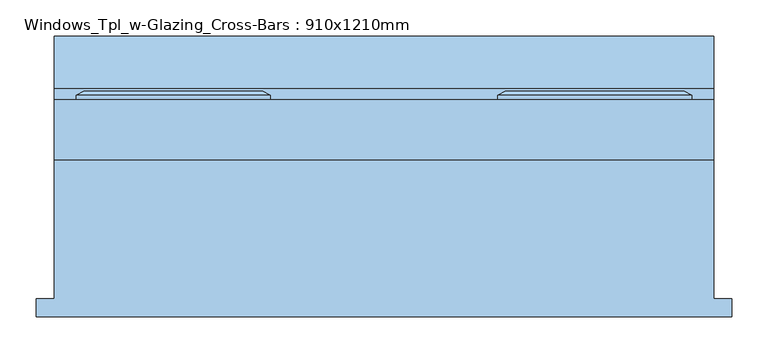
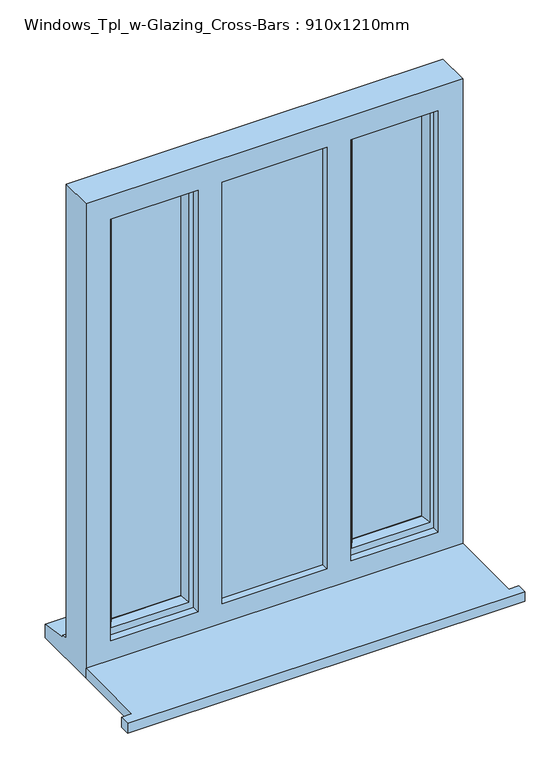
"""IFC4 building model written with IfcOpenShell, lengths in millimetres: window geometry, Windows_Tpl_w-Glazing_Cross-Bars : 910x1210mm."""

from ifc_helpers import new_model, si_unit, frame, origin, place, context, project, spatial, polyline, outline, extrude, faceted_brep, source, transform, mapped, element, save


def windows_tpl_w_glazing_cross_bars_910x1210mm_b9cba8ba(model_context):
    return source(origin(), model_context, "Body", "SolidModel", [
        extrude(outline(polyline([(-906.6666667, -178.7934322), (-906.6666667, -153.7934322), (-881.6666667, -153.7934322), (-881.6666667, 37.7065678), (28.3333333, 37.7065678), (28.3333333, -153.7934322), (53.3333333, -153.7934322), (53.3333333, -178.7934322), (-906.6666667, -178.7934322)])), frame((0.0, 0.0, 900.0), z_axis=(0.0, 0.0, 1.0), x_axis=(1.0, 0.0, 0.0)), (0.0, 0.0, 1.0), 25.0),
        extrude(outline(polyline([(-623.3333333, 72.4565678), (-811.6666667, 72.4565678), (-811.6666667, 96.4565678), (-623.3333333, 96.4565678), (-623.3333333, 72.4565678)])), frame((0.0, 0.0, 993.0), z_axis=(0.0, 0.0, 1.0), x_axis=(1.0, 0.0, 0.0)), (0.0, 0.0, 1.0), 1047.0),
        extrude(outline(polyline([(-41.5186289, 72.4565678), (-230.1480377, 72.4565678), (-230.1480377, 96.4565678), (-41.5186289, 96.4565678), (-41.5186289, 72.4565678)])), frame((0.0, 0.0, 992.8519623), z_axis=(0.0, 0.0, 1.0), x_axis=(1.0, 0.0, 0.0)), (0.0, 0.0, 1.0), 1047.2960754),
        extrude(outline(polyline([(-563.3333333, 79.7065678), (-290.0, 79.7065678), (-290.0, 55.7065678), (-563.3333333, 55.7065678), (-563.3333333, 79.7065678)])), frame((0.0, 0.0, 963.0), z_axis=(0.0, 0.0, 1.0), x_axis=(1.0, 0.0, 0.0)), (0.0, 0.0, 1.0), 1107.0),
        faceted_brep([(28.3333333, 37.7065678, 2110.0), (-881.6666667, 37.7065678, 2110.0), (-881.6666667, 37.7065678, 900.0), (28.3333333, 37.7065678, 900.0), (-31.6666667, 37.7065678, 2050.0), (-31.6666667, 37.7065678, 975.0), (-242.0, 37.7065678, 975.0), (-242.0, 37.7065678, 2050.0), (-300.0, 37.7065678, 2050.0), (-300.0, 37.7065678, 975.0), (-553.3333333, 37.7065678, 975.0), (-553.3333333, 37.7065678, 2050.0), (-611.3333333, 37.7065678, 2050.0), (-611.3333333, 37.7065678, 975.0), (-821.6666667, 37.7065678, 975.0), (-821.6666667, 37.7065678, 2050.0), (-881.6666667, 120.7065678, 2110.0), (-881.6666667, 120.7065678, 951.0), (-881.6666667, 135.7065678, 949.68767), (-881.6666667, 135.7065678, 944.7449676), (-881.6666667, 208.2065678, 933.8088847), (-881.6666667, 208.2065678, 900.0), (28.3333333, 120.7065678, 2110.0), (28.3333333, 120.7065678, 951.0), (-841.6666667, 120.7065678, 2070.0), (-841.6666667, 120.7065678, 963.0), (-593.3333333, 120.7065678, 963.0), (-593.3333333, 120.7065678, 2070.0), (-553.3333333, 120.7065678, 2070.0), (-553.3333333, 120.7065678, 963.0), (-300.0, 120.7065678, 963.0), (-300.0, 120.7065678, 2070.0), (-260.0, 120.7065678, 2070.0), (-260.0, 120.7065678, 963.0), (-11.6666667, 120.7065678, 963.0), (-11.6666667, 120.7065678, 2070.0), (-841.6666667, 55.7065678, 2070.0), (-841.6666667, 55.7065678, 963.0), (-563.3333333, 55.7065678, 2070.0), (-290.0, 55.7065678, 2070.0), (-290.0, 55.7065678, 963.0), (-563.3333333, 55.7065678, 963.0), (-300.0, 55.7065678, 2050.0), (-553.3333333, 55.7065678, 2050.0), (-553.3333333, 55.7065678, 975.0), (-300.0, 55.7065678, 975.0), (-260.0, 55.7065678, 2070.0), (-11.6666667, 55.7065678, 2070.0), (-11.6666667, 55.7065678, 963.0), (-260.0, 55.7065678, 963.0), (-31.6666667, 55.7065678, 2050.0), (-242.0, 55.7065678, 2050.0), (-242.0, 55.7065678, 975.0), (-31.6666667, 55.7065678, 975.0), (-593.3333333, 55.7065678, 2070.0), (-593.3333333, 55.7065678, 963.0), (-611.3333333, 55.7065678, 2050.0), (-821.6666667, 55.7065678, 2050.0), (-821.6666667, 55.7065678, 975.0), (-611.3333333, 55.7065678, 975.0), (-553.3333333, 79.7065678, 2070.0), (-300.0, 79.7065678, 2070.0), (-290.0, 79.7065678, 2070.0), (-563.3333333, 79.7065678, 2070.0), (28.3333333, 208.2065678, 900.0), (28.3333333, 208.2065678, 933.8088847), (28.3333333, 135.7065678, 944.7449676), (28.3333333, 135.7065678, 949.68767), (-553.3333333, 79.7065678, 963.0), (-563.3333333, 79.7065678, 963.0), (-290.0, 79.7065678, 963.0), (-300.0, 79.7065678, 963.0)], [[[0, 1, 2, 3], [4, 5, 6, 7], [8, 9, 10, 11], [12, 13, 14, 15]], [[2, 1, 16, 17, 18, 19, 20, 21]], [[17, 16, 22, 23], [24, 25, 26, 27], [28, 29, 30, 31], [32, 33, 34, 35]], [[25, 24, 36, 37]], [[38, 39, 40, 41], [42, 43, 44, 45]], [[46, 47, 48, 49], [50, 51, 52, 53]], [[36, 54, 55, 37], [56, 57, 58, 59]], [[57, 15, 14, 58]], [[1, 0, 22, 16]], [[36, 24, 27, 54]], [[35, 47, 46, 32]], [[60, 28, 31, 61, 62, 39, 38, 63]], [[15, 57, 56, 12]], [[50, 4, 7, 51]], [[11, 43, 42, 8]], [[23, 22, 0, 3, 64, 65, 66, 67]], [[35, 34, 48, 47]], [[4, 50, 53, 5]], [[43, 11, 10, 44]], [[12, 56, 59, 13]], [[27, 26, 55, 54]], [[29, 28, 60, 68]], [[68, 60, 63, 69]], [[69, 63, 38, 41]], [[62, 70, 40, 39]], [[70, 62, 61, 71]], [[71, 61, 31, 30]], [[33, 32, 46, 49]], [[51, 7, 6, 52]], [[8, 42, 45, 9]], [[64, 3, 2, 21]], [[65, 64, 21, 20]], [[66, 65, 20, 19]], [[67, 66, 19, 18]], [[23, 67, 18, 17]], [[26, 25, 37, 55]], [[34, 33, 49, 48]], [[41, 40, 70, 71, 30, 29, 68, 69]], [[6, 5, 53, 52]], [[45, 44, 10, 9]], [[59, 58, 14, 13]]]),
        extrude(outline(polyline([(963.0, -436.6666667), (963.0, -416.6666667), (1506.5, -416.6666667), (1506.5, -290.0), (1526.5, -290.0), (1526.5, -416.6666667), (2070.0, -416.6666667), (2070.0, -436.6666667), (1526.5, -436.6666667), (1526.5, -563.3333333), (1506.5, -563.3333333), (1506.5, -436.6666667), (963.0, -436.6666667)])), frame((0.0, 63.7065678, 0.0), z_axis=(0.0, 1.0, 0.0), x_axis=(0.0, 0.0, 1.0)), (0.0, 0.0, 1.0), 8.0),
        extrude(outline(polyline([(993.0, -145.8333333), (993.0, -125.8333333), (1506.5, -125.8333333), (1506.5, -41.6666667), (1526.5, -41.6666667), (1526.5, -125.8333333), (2040.1480377, -125.8333333), (2040.1480377, -145.8333333), (1526.5, -145.8333333), (1526.5, -230.1480377), (1506.5, -230.1480377), (1506.5, -145.8333333), (993.0, -145.8333333)])), frame((0.0, 92.7065678, 0.0), z_axis=(0.0, 1.0, 0.0), x_axis=(0.0, 0.0, 1.0)), (0.0, 0.0, 1.0), 8.0),
        extrude(outline(polyline([(993.0, -727.5), (993.0, -707.5), (1506.5, -707.5), (1506.5, -623.3333333), (1526.5, -623.3333333), (1526.5, -707.5), (2040.1480377, -707.5), (2040.1480377, -727.5), (1526.5, -727.5), (1526.5, -811.6666667), (1506.5, -811.6666667), (1506.5, -727.5), (993.0, -727.5)])), frame((0.0, 92.7065678, 0.0), z_axis=(0.0, 1.0, 0.0), x_axis=(0.0, 0.0, 1.0)), (0.0, 0.0, 1.0), 8.0),
        faceted_brep([(-583.3333333, 120.7065678, 2080.0), (-583.3333333, 126.4800705, 2080.0), (-851.6666667, 126.4800705, 2080.0), (-851.6666667, 120.7065678, 2080.0), (-593.3333333, 55.7065678, 2070.0), (-593.3333333, 120.7065678, 2070.0), (-841.6666667, 120.7065678, 2070.0), (-841.6666667, 55.7065678, 2070.0), (-633.3333333, 70.1994677, 2030.0), (-623.1852956, 55.7065678, 2040.1480377), (-811.8147044, 55.7065678, 2040.1480377), (-801.6666667, 70.1994677, 2030.0), (-633.3333333, 84.7065678, 2030.0), (-801.6666667, 84.7065678, 2030.0), (-623.3333333, 108.7065678, 2040.0), (-623.3333333, 84.7065678, 2040.0), (-811.6666667, 84.7065678, 2040.0), (-811.6666667, 108.7065678, 2040.0), (-633.3333333, 126.4800705, 2030.0), (-633.3333333, 108.7065678, 2030.0), (-801.6666667, 108.7065678, 2030.0), (-801.6666667, 126.4800705, 2030.0), (-615.8875785, 132.2535732, 2047.4457548), (-819.1124215, 132.2535732, 2047.4457548), (-594.117943, 132.2535732, 2069.2153903), (-840.882057, 132.2535732, 2069.2153903), (-851.6666667, 126.4800705, 953.0), (-851.6666667, 120.7065678, 953.0), (-841.6666667, 120.7065678, 963.0), (-841.6666667, 55.7065678, 963.0), (-811.8147044, 55.7065678, 992.8519623), (-801.6666667, 70.1994677, 1003.0), (-801.6666667, 84.7065678, 1003.0), (-811.6666667, 84.7065678, 993.0), (-811.6666667, 108.7065678, 993.0), (-801.6666667, 108.7065678, 1003.0), (-801.6666667, 126.4800705, 1003.0), (-819.1124215, 132.2535732, 985.5542452), (-840.882057, 132.2535732, 963.7846097), (-583.3333333, 126.4800705, 953.0), (-583.3333333, 120.7065678, 953.0), (-593.3333333, 120.7065678, 963.0), (-593.3333333, 55.7065678, 963.0), (-623.1852956, 55.7065678, 992.8519623), (-633.3333333, 70.1994677, 1003.0), (-633.3333333, 84.7065678, 1003.0), (-623.3333333, 84.7065678, 993.0), (-623.3333333, 108.7065678, 993.0), (-633.3333333, 108.7065678, 1003.0), (-633.3333333, 126.4800705, 1003.0), (-615.8875785, 132.2535732, 985.5542452), (-594.117943, 132.2535732, 963.7846097)], [[[0, 1, 2, 3]], [[4, 5, 6, 7]], [[8, 9, 10, 11]], [[12, 8, 11, 13]], [[14, 15, 16, 17]], [[18, 19, 20, 21]], [[22, 18, 21, 23]], [[1, 24, 25, 2]], [[3, 2, 26, 27]], [[7, 6, 28, 29]], [[11, 10, 30, 31]], [[13, 11, 31, 32]], [[17, 16, 33, 34]], [[21, 20, 35, 36]], [[23, 21, 36, 37]], [[2, 25, 38, 26]], [[27, 26, 39, 40]], [[0, 3, 27, 40], [41, 28, 6, 5]], [[29, 28, 41, 42]], [[4, 7, 29, 42], [43, 30, 10, 9]], [[31, 30, 43, 44]], [[32, 31, 44, 45]], [[46, 33, 16, 15], [12, 13, 32, 45]], [[34, 33, 46, 47]], [[14, 17, 34, 47], [48, 35, 20, 19]], [[36, 35, 48, 49]], [[37, 36, 49, 50]], [[51, 38, 25, 24], [22, 23, 37, 50]], [[26, 38, 51, 39]], [[40, 39, 1, 0]], [[42, 41, 5, 4]], [[44, 43, 9, 8]], [[45, 44, 8, 12]], [[47, 46, 15, 14]], [[49, 48, 19, 18]], [[50, 49, 18, 22]], [[39, 51, 24, 1]]]),
        faceted_brep([(-270.0, 120.7065678, 2080.0), (-270.0, 126.4800705, 2080.0), (-270.0, 126.4800705, 953.0), (-270.0, 120.7065678, 953.0), (-260.0, 55.7065678, 2070.0), (-260.0, 120.7065678, 2070.0), (-260.0, 120.7065678, 963.0), (-260.0, 55.7065678, 963.0), (-220.0, 70.1994677, 2030.0), (-230.1480377, 55.7065678, 2040.1480377), (-230.1480377, 55.7065678, 992.8519623), (-220.0, 70.1994677, 1003.0), (-220.0, 84.7065678, 2030.0), (-220.0, 84.7065678, 1003.0), (-230.0, 108.7065678, 2040.0), (-230.0, 84.7065678, 2040.0), (-230.0, 84.7065678, 993.0), (-230.0, 108.7065678, 993.0), (-220.0, 126.4800705, 2030.0), (-220.0, 108.7065678, 2030.0), (-220.0, 108.7065678, 1003.0), (-220.0, 126.4800705, 1003.0), (-237.4457548, 132.2535732, 2047.4457548), (-237.4457548, 132.2535732, 985.5542452), (-259.2153903, 132.2535732, 2069.2153903), (-259.2153903, 132.2535732, 963.7846097), (-1.6666667, 126.4800705, 953.0), (-1.6666667, 120.7065678, 953.0), (-11.6666667, 120.7065678, 963.0), (-11.6666667, 55.7065678, 963.0), (-41.5186289, 55.7065678, 992.8519623), (-51.6666667, 70.1994677, 1003.0), (-51.6666667, 84.7065678, 1003.0), (-41.6666667, 84.7065678, 993.0), (-41.6666667, 108.7065678, 993.0), (-51.6666667, 108.7065678, 1003.0), (-51.6666667, 126.4800705, 1003.0), (-34.2209119, 132.2535732, 985.5542452), (-12.4512764, 132.2535732, 963.7846097), (-1.6666667, 126.4800705, 2080.0), (-1.6666667, 120.7065678, 2080.0), (-11.6666667, 120.7065678, 2070.0), (-11.6666667, 55.7065678, 2070.0), (-41.5186289, 55.7065678, 2040.1480377), (-51.6666667, 70.1994677, 2030.0), (-51.6666667, 84.7065678, 2030.0), (-41.6666667, 84.7065678, 2040.0), (-41.6666667, 108.7065678, 2040.0), (-51.6666667, 108.7065678, 2030.0), (-51.6666667, 126.4800705, 2030.0), (-34.2209119, 132.2535732, 2047.4457548), (-12.4512764, 132.2535732, 2069.2153903)], [[[0, 1, 2, 3]], [[4, 5, 6, 7]], [[8, 9, 10, 11]], [[12, 8, 11, 13]], [[14, 15, 16, 17]], [[18, 19, 20, 21]], [[22, 18, 21, 23]], [[1, 24, 25, 2]], [[3, 2, 26, 27]], [[7, 6, 28, 29]], [[11, 10, 30, 31]], [[13, 11, 31, 32]], [[17, 16, 33, 34]], [[21, 20, 35, 36]], [[23, 21, 36, 37]], [[2, 25, 38, 26]], [[27, 26, 39, 40]], [[29, 28, 41, 42]], [[31, 30, 43, 44]], [[32, 31, 44, 45]], [[34, 33, 46, 47]], [[36, 35, 48, 49]], [[37, 36, 49, 50]], [[26, 38, 51, 39]], [[40, 39, 1, 0]], [[3, 27, 40, 0], [5, 41, 28, 6]], [[42, 41, 5, 4]], [[7, 29, 42, 4], [9, 43, 30, 10]], [[44, 43, 9, 8]], [[45, 44, 8, 12]], [[15, 46, 33, 16], [13, 32, 45, 12]], [[47, 46, 15, 14]], [[17, 34, 47, 14], [19, 48, 35, 20]], [[49, 48, 19, 18]], [[50, 49, 18, 22]], [[24, 51, 38, 25], [23, 37, 50, 22]], [[39, 51, 24, 1]]]),
    ])


if __name__ == "__main__":
    model = new_model("IFC4")
    model_context = context("Model", 3, world=origin())
    ifc_project = project(units=[si_unit("LENGTHUNIT", "METRE", prefix="MILLI")], contexts=[model_context])
    site = spatial("IfcSite", under=ifc_project)
    building = spatial("IfcBuilding", under=site)
    placement = place(None, origin())
    windows_tpl_w_glazing_cross_bars_910x1210mm_shape = windows_tpl_w_glazing_cross_bars_910x1210mm_b9cba8ba(model_context)
    element("IfcWindow", 1, ObjectType="Windows_Tpl_w-Glazing_Cross-Bars : 910x1210mm", at=placement, inside=building, context=model_context, shape_type="MappedRepresentation", body=[
        mapped(windows_tpl_w_glazing_cross_bars_910x1210mm_shape, transform((0.0, 0.0, 0.0), x_axis=(1.0, 0.0, 0.0), y_axis=(0.0, 1.0, 0.0), z_axis=(0.0, 0.0, 1.0))),
    ])
    save(model, "model.ifc")

# Revit data of these elements
# Type "Windows_Tpl_w-Glazing_Cross-Bars : 910x1210mm"
#   Type Mark = "51"
#   Operation = "TriplePanelVertical"
#   Construction Type Id = "GSP4R"
#   Manufacturer = "Revit"
#   Keynote = "L10"
#   Analytic Construction = "1/8 in Pilkington single glazing"
#   Wrap Layers (Ext) from Ext = 102.5 mm
#   Wrap Layers (Int) from Ext = 177.5 mm
#   Window Board Projection = 25 mm
#   Window Board Extension = 25 mm
#   Visual Light Transmittance = 0.9
#   Solar Heat Gain Coefficient = 0.78
#   Rough Width = 910 mm
#   Rough Height = 1210 mm
#   Height = 1210 mm
#   Width = 910 mm
#   Heat Transfer Coefficient (U) = 3.6886 W/(m²·K)
#   Glazing Thickness = 24 mm
#   Glazing Bar Thickness = 20 mm
#   FrameOffset - External = 50 mm
#   Frame Depth = 65 mm
#   Default Head Height = 2110 mm
#   Cill Depth = 87.5 mm
#   Cavity Closer Width = 50 mm
#   Cavity Closer Offset from Ext = 102.5 mm
#   Cavity Closer Depth = 85 mm
#   Vis - Glazing Bars = yes
#   Vis - Cavity Closers = yes
#   Material Trim = Window Frame
#   Material Glazing Bars = Window Frame
#   Material Glass = Glass
#   Material Frame = Window Frame
#   Wall Closure = (empty or 0)
# Element 1 (IfcWindow, "Windows_Tpl_w-Glazing_Cross-Bars : 910x1210mm")
#   Materials on its faces: "Window Frame", "Glass"
# Materials
#   "Window Frame": class "Miscellaneous", colour RGB 249 249 249, transparency 0, Keynote = "L10"
#   "Glass": class "Glass", colour RGB 0 128 192, transparency 0.9, Description = "Soda Lime Glass", Cost = 0
